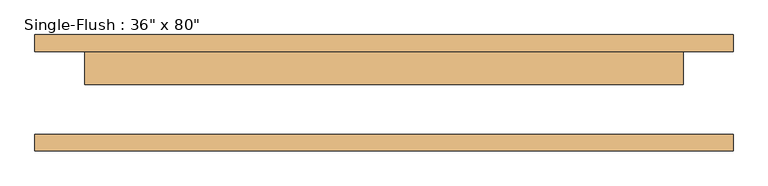
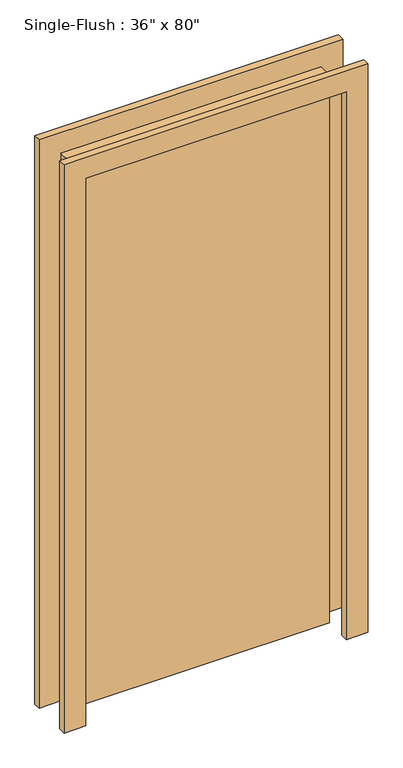
"""IFC4 building model written with IfcOpenShell, lengths in millimetres: door geometry."""

from ifc_helpers import new_model, si_unit, frame, origin, origin_with_axes, place, context, project, spatial, polyline, outline, extrude, source, transform, mapped, element, save


def door_bc81e0a2(model_context):
    return source(origin(), model_context, "Body", "SweptSolid", [
        extrude(outline(polyline([(2108.2, -533.4), (0.0, -533.4), (0.0, -457.2), (2032.0, -457.2), (2032.0, 457.2), (0.0, 457.2), (0.0, 533.4), (2108.2, 533.4), (2108.2, -533.4)])), frame((0.0, 63.5, 0.0), z_axis=(0.0, 1.0, 0.0), x_axis=(0.0, 0.0, 1.0)), (0.0, 0.0, 1.0), 25.4),
        extrude(outline(polyline([(2108.2, 533.4), (2108.2, -533.4), (0.0, -533.4), (0.0, -457.2), (2032.0, -457.2), (2032.0, 457.2), (0.0, 457.2), (0.0, 533.4), (2108.2, 533.4)])), frame((0.0, -88.9, 0.0), z_axis=(0.0, 1.0, 0.0), x_axis=(0.0, 0.0, 1.0)), (0.0, 0.0, 1.0), 25.4),
        extrude(outline(polyline([(457.2, 12.7), (-457.2, 12.7), (-457.2, 63.5), (457.2, 63.5), (457.2, 12.7)])), origin_with_axes(), (0.0, 0.0, 1.0), 2032.0),
    ])


if __name__ == "__main__":
    model = new_model("IFC4")
    model_context = context("Model", 3, world=origin())
    ifc_project = project(units=[si_unit("LENGTHUNIT", "METRE", prefix="MILLI")], contexts=[model_context])
    site = spatial("IfcSite", under=ifc_project)
    building = spatial("IfcBuilding", under=site)
    placement = place(None, origin())
    door_shape = door_bc81e0a2(model_context)
    element("IfcDoor", 1, ObjectType="Single-Flush : 36\" x 80\"", at=placement, inside=building, context=model_context, shape_type="MappedRepresentation", body=[
        mapped(door_shape, transform((0.0, 0.0, 0.0), x_axis=(1.0, 0.0, 0.0), y_axis=(0.0, 1.0, 0.0), z_axis=(0.0, 0.0, 1.0))),
    ])
    save(model, "model.ifc")

# Revit data of these elements
# Type "Single-Flush : 36\" x 80\""
#   Type Mark = "6"
#   Construction Type Id = "MDOOR"
#   Assembly Code = "C1020"
#   Analytic Construction = "Metal"
#   Thickness = 0.0508 m
#   Heat Transfer Coefficient (U) = 3.7021 W/(m²·K)
#   Height = 2.032 m
#   Trim Projection Ext = 0.0254 m
#   Trim Projection Int = 0.0254 m
#   Trim Width = 0.0762 m
#   Width = 0.9144 m
#   Define Thermal Properties by = 1
#   Door Material = Door - Panel
#   Frame Material = Door - Frame
#   Visual Light Transmittance = 0
#   Solar Heat Gain Coefficient = 0
#   Function = (empty or 0)
#   Wall Closure = (empty or 0)
# Element 1 (IfcDoor, "Single-Flush : 36\" x 80\"")
#   Materials on its faces: "Door - Frame", "Door - Panel"
# Materials
#   "Door - Panel": class "Wood", colour RGB 210 159 95, transparency 0, Cost = 0
#   "Door - Frame": class "Miscellaneous", colour RGB 118 70 51, transparency 0, Cost = 0
